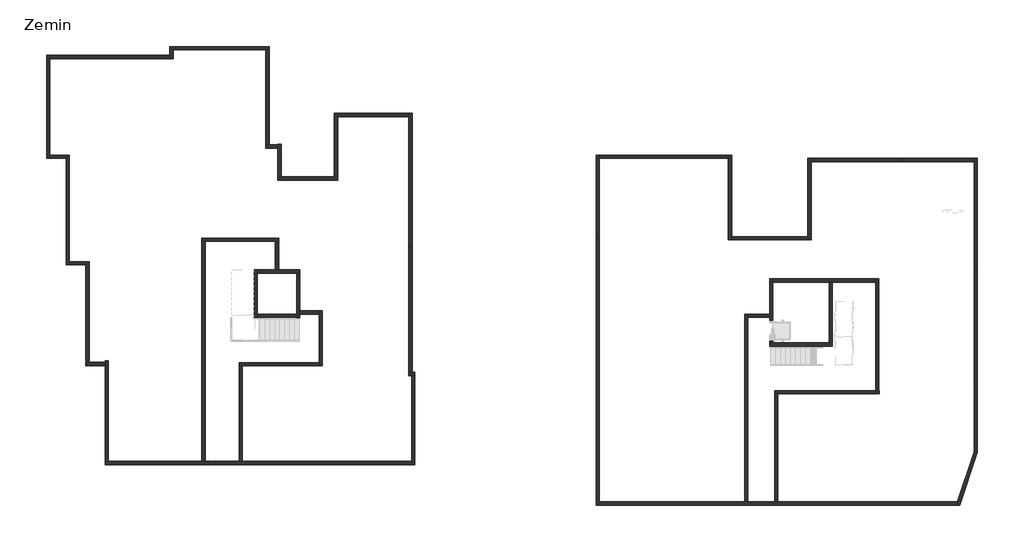
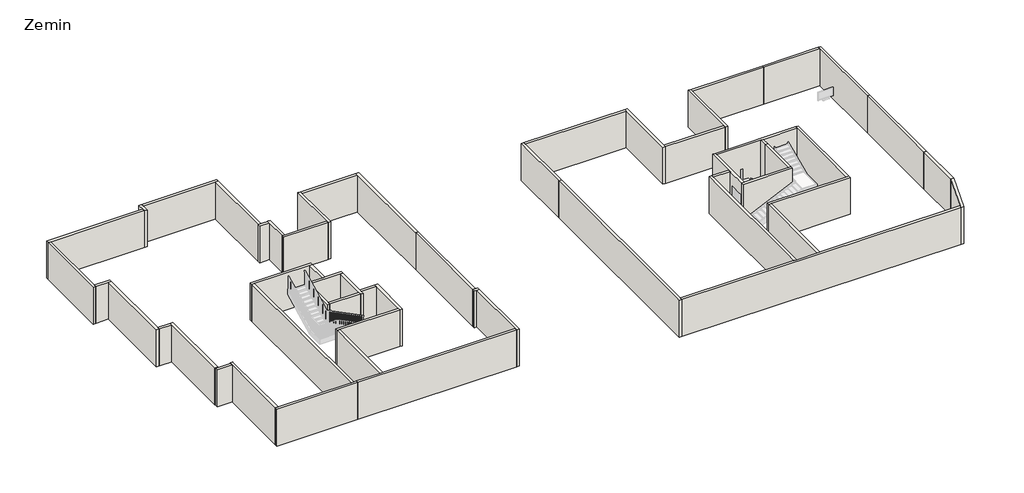
# One storey, part 1 of 2: 56 walls.
# Revit data of these elements (continued)
# Room, not placed, phase "New Construction", upper offset 0 cm, lower offset 0 cm
#   Number = "143"
#   Name = "Room"
# Room, not placed, phase "New Construction", upper offset 0 cm, lower offset 0 cm
#   Number = "144"
#   Name = "Room"
# Room, not placed, phase "New Construction", upper offset 0 cm, lower offset 0 cm
#   Number = "145"
#   Name = "Room"
# Room, not placed, phase "New Construction", upper offset 0 cm, lower offset 0 cm
#   Number = "146"
#   Name = "Room"
# Area, not placed, upper offset 0 cm, lower offset 0 cm
#   Number = "8"
#   Name = "Dere Parsel Toplam Alan"
# Room, not placed, phase "New Construction", upper offset 0 cm, lower offset 0 cm
#   Number = "108"
#   Name = "ASANSÖR"
# Room, not placed, phase "New Construction", upper offset 0 cm, lower offset 0 cm
#   Number = "89"
#   Name = "Room"
# Room, not placed, phase "New Construction", upper offset 0 cm, lower offset 0 cm
#   Number = "147"
#   Name = "Room"
# Room, not placed, phase "New Construction", upper offset 0 cm, lower offset 0 cm
#   Number = "19"
#   Name = "Room"
# Room, not placed, phase "New Construction", upper offset 0 cm, lower offset 0 cm
#   Number = ""
#   Name = ""
# Room, not placed, phase "New Construction", upper offset 0 cm, lower offset 0 cm
#   Number = "21"
#   Name = "Room"
# Room, not placed, phase "New Construction", upper offset 0 cm, lower offset 0 cm
#   Number = "22"
#   Name = "Room"
# Room, not placed, phase "New Construction", upper offset 0 cm, lower offset 0 cm
#   Number = "23"
#   Name = "Room"
# Room, not placed, phase "New Construction", upper offset 0 cm, lower offset 0 cm
#   Number = "24"
#   Name = "Room"
# Room, not placed, phase "New Construction", upper offset 0 cm, lower offset 0 cm
#   Number = "25"
#   Name = "Room"
# Room, not placed, phase "New Construction", upper offset 0 cm, lower offset 0 cm
#   Number = "64"
#   Name = "Room"
# Room, not placed, phase "New Construction", upper offset 0 cm, lower offset 0 cm
#   Number = "65"
#   Name = "Room"
# Room, not placed, phase "New Construction", upper offset 0 cm, lower offset 0 cm
#   Number = "66"
#   Name = "Room"
# Room, not placed, phase "New Construction", upper offset 0 cm, lower offset 0 cm
#   Number = ""
#   Name = ""
# Room, not placed, phase "New Construction", upper offset 0 cm, lower offset 0 cm
#   Number = "27"
#   Name = "Room"
# Room, not placed, phase "New Construction", upper offset 0 cm, lower offset 0 cm
#   Number = "42"
#   Name = "Room"
# Area, not placed, upper offset 0 cm, lower offset 0 cm
#   Number = "13"
#   Name = "Area"
# Area, not placed, upper offset 0 cm, lower offset 0 cm
#   Number = "14"
#   Name = "Area"
# Area, not placed, upper offset 0 cm, lower offset 0 cm
#   Number = "2"
#   Name = "Area"
# Room, not placed, phase "New Construction", upper offset 0 cm, lower offset 0 cm
#   Number = "43"
#   Name = "Room"
# Room, not placed, phase "New Construction", upper offset 0 cm, lower offset 0 cm
#   Number = ""
#   Name = ""
# Room, not placed, phase "New Construction", upper offset 0 cm, lower offset 0 cm
#   Number = "94"
#   Name = "Room"
# Room, not placed, phase "New Construction", upper offset 0 cm, lower offset 0 cm
#   Number = ""
#   Name = ""
# Area at (12167.029, -1298.394) mm, upper offset 243.84 cm, lower offset 0 cm
#   Number = "17"
#   Name = "Area"
# Room, not placed, phase "New Construction", upper offset 0 cm, lower offset 0 cm
#   Number = "136"
#   Name = "Room"
# Room, not placed, phase "New Construction", upper offset 0 cm, lower offset 0 cm
#   Number = "1"
#   Name = "Room"
# Area, not placed, upper offset 0 cm, lower offset 0 cm
#   Number = "3"
#   Name = "Area"
# Room, not placed, phase "New Construction", upper offset 0 cm, lower offset 0 cm
#   Number = "7"
#   Name = "Room"
# Room, not placed, phase "New Construction", upper offset 0 cm, lower offset 0 cm
#   Number = "8"
#   Name = "Room"
# Area at (-17506.584, 6793.532) mm, upper offset 243.84 cm, lower offset 0 cm
#   Number = "18"
#   Name = "Area"
# Room, not placed, phase "New Construction", upper offset 0 cm, lower offset 0 cm
#   Number = "2"
#   Name = "Room"
# Room, not placed, phase "New Construction", upper offset 0 cm, lower offset 0 cm
#   Number = "46"
#   Name = "Room"
# Room, not placed, phase "New Construction", upper offset 0 cm, lower offset 0 cm
#   Number = "3"
#   Name = "Room"
# Room, not placed, phase "New Construction", upper offset 0 cm, lower offset 0 cm
#   Number = ""
#   Name = ""
# Room, not placed, phase "New Construction", upper offset 0 cm, lower offset 0 cm
#   Number = "4"
#   Name = "Room"
# Area, not placed, upper offset 0 cm, lower offset 0 cm
#   Number = "1"
#   Name = "Area"
# Room, not placed, phase "New Construction", upper offset 0 cm, lower offset 0 cm
#   Number = ""
#   Name = ""
# Room, not placed, phase "New Construction", upper offset 0 cm, lower offset 0 cm
#   Number = "29"
#   Name = "Room"
# Area, not placed, upper offset 0 cm, lower offset 0 cm
#   Number = "7"
#   Name = "Dere Parsel Toplam Alan"
# Room, not placed, phase "New Construction", upper offset 0 cm, lower offset 0 cm
#   Number = "95"
#   Name = "ASANSÖR"
# Room, not placed, phase "New Construction", upper offset 0 cm, lower offset 0 cm
#   Number = "96"
#   Name = "Room"
# Room, not placed, phase "New Construction", upper offset 0 cm, lower offset 0 cm
#   Number = "97"
#   Name = "7"
# Room, not placed, phase "New Construction", upper offset 0 cm, lower offset 0 cm
#   Number = "98"
#   Name = "8"
# Room, not placed, phase "New Construction", upper offset 0 cm, lower offset 0 cm
#   Number = "99"
#   Name = "9"
# Room, not placed, phase "New Construction", upper offset 0 cm, lower offset 0 cm
#   Number = "100"
#   Name = "1"
# Room, not placed, phase "New Construction", upper offset 0 cm, lower offset 0 cm
#   Number = "101"
#   Name = "5"
# Room, not placed, phase "New Construction", upper offset 0 cm, lower offset 0 cm
#   Number = "102"
#   Name = "2"
# Room, not placed, phase "New Construction", upper offset 0 cm, lower offset 0 cm
#   Number = "103"
#   Name = "4"
# Room, not placed, phase "New Construction", upper offset 0 cm, lower offset 0 cm
#   Number = "104"
#   Name = "3"
# Room, not placed, phase "New Construction", upper offset 0 cm, lower offset 0 cm
#   Number = "105"
#   Name = "6"
